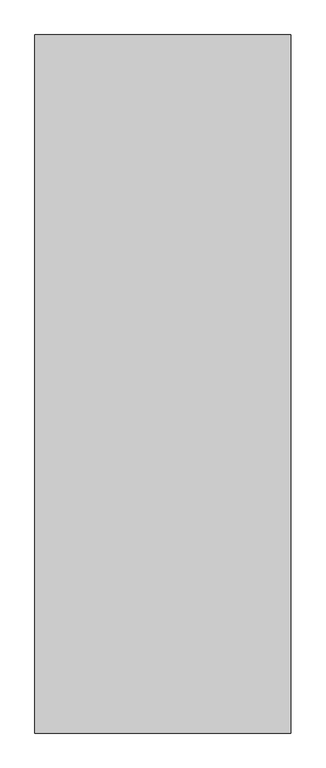
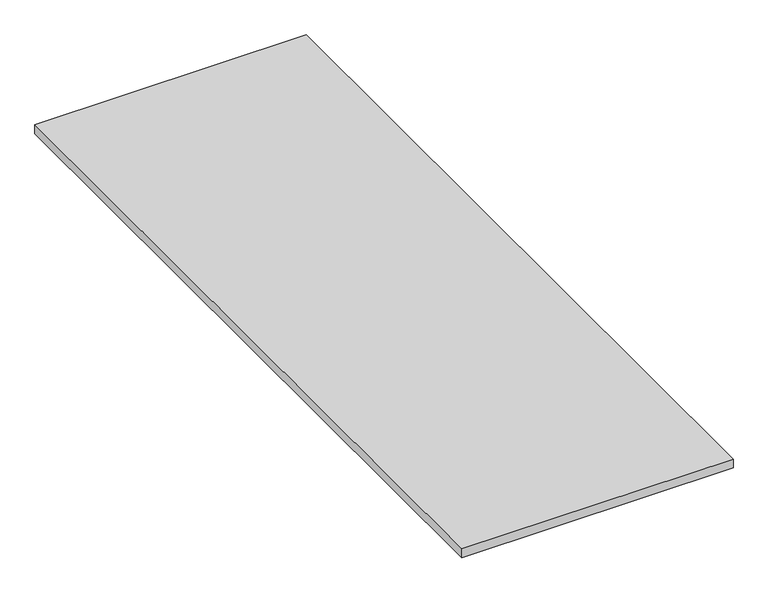
"""IFC4 building model written with IfcOpenShell, lengths in millimetres: proxy geometry, Plywood065 181 : Plywood065 181."""

from ifc_helpers import new_model, si_unit, frame, origin, place, context, project, spatial, polyline, outline, extrude, source, transform, mapped, element, save


def generic_models_804268d1(model_context):
    return source(origin(), model_context, "Body", "SweptSolid", [
        extrude(outline(polyline([(-8768.1487014, 7982.1529359), (-9501.5737014, 7982.1529359), (-9501.5737014, 9982.1529359), (-8768.1487014, 9982.1529359), (-8768.1487014, 7982.1529359)])), frame((0.0, 0.0, 32568.8960253), z_axis=(0.0, 0.0, 1.0), x_axis=(1.0, 0.0, 0.0)), (0.0, 0.0, 1.0), 25.4),
    ])


if __name__ == "__main__":
    model = new_model("IFC4")
    model_context = context("Model", 3, world=origin())
    ifc_project = project(units=[si_unit("LENGTHUNIT", "METRE", prefix="MILLI")], contexts=[model_context])
    site = spatial("IfcSite", under=ifc_project)
    building = spatial("IfcBuilding", under=site)
    placement = place(None, origin())
    generic_models_shape = generic_models_804268d1(model_context)
    element("IfcBuildingElementProxy", 1, Name="Plywood065 181 : Plywood065 181", ObjectType="Plywood065 181 : Plywood065 181", at=placement, inside=building, context=model_context, shape_type="MappedRepresentation", body=[
        mapped(generic_models_shape, transform((0.0, 0.0, 0.0), x_axis=(1.0, 0.0, 0.0), y_axis=(0.0, 1.0, 0.0), z_axis=(0.0, 0.0, 1.0))),
    ])
    save(model, "model.ifc")

# Revit data of these elements
# Type "Plywood065 181 : Plywood065 181"
#   NameOverride = "Plywood065"
# Element 1 (IfcBuildingElementProxy, "Plywood065 181 : Plywood065 181")
#   Materials on its faces: "CDX PLYWOOD - SEE STRUCTURAL DWGS"
# Materials
#   "CDX PLYWOOD - SEE STRUCTURAL DWGS": class "Unassigned", colour RGB 177 130 114, transparency 0, Cost = 0
